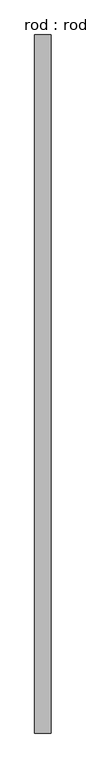
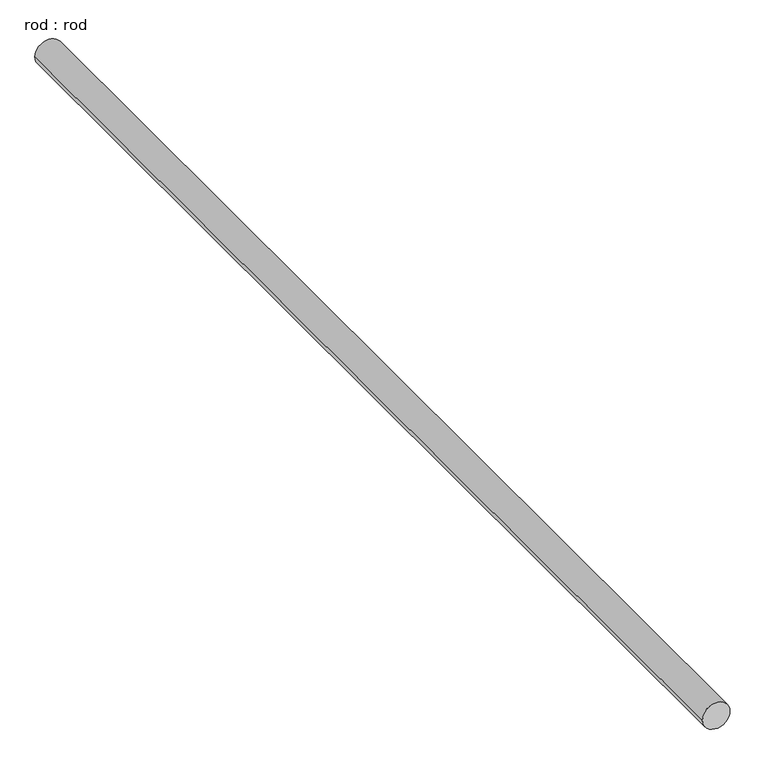
"""IFC4 building model written with IfcOpenShell, lengths in millimetres: proxy geometry, rod : rod."""

from ifc_helpers import new_model, si_unit, point, frame, frame_2d, origin, place, context, project, spatial, circle_curve, trimmed, segment, composite_curve, outline, extrude, source, transform, mapped, element, save


def rod_rod_caa43e47(model_context):
    return source(origin(), model_context, "Body", "SweptSolid", [
        extrude(outline(composite_curve([segment(trimmed(circle_curve(frame_2d((0.0108462, 0.0)), 200.0), [point((0.0108462, 200.0))], [point((0.0108462, -200.0))], False, "CARTESIAN"), True, "CONTINUOUS"), segment(trimmed(circle_curve(frame_2d((0.0108462, 0.0)), 200.0), [point((0.0108462, -200.0))], [point((0.0108462, 200.0))], False, "CARTESIAN"), True, "CONTINUOUS")], self_intersect=False)), frame((0.0, -4343.1908587, 0.0), z_axis=(0.0, 1.0, 0.0), x_axis=(0.0, 0.0, 1.0)), (0.0, 0.0, 1.0), 16871.8389481),
    ])


if __name__ == "__main__":
    model = new_model("IFC4")
    model_context = context("Model", 3, world=origin())
    ifc_project = project(units=[si_unit("LENGTHUNIT", "METRE", prefix="MILLI")], contexts=[model_context])
    site = spatial("IfcSite", under=ifc_project)
    building = spatial("IfcBuilding", under=site)
    placement = place(None, origin())
    rod_rod_shape = rod_rod_caa43e47(model_context)
    element("IfcBuildingElementProxy", 1, Name="rod : rod", ObjectType="rod : rod", at=placement, inside=building, context=model_context, shape_type="MappedRepresentation", body=[
        mapped(rod_rod_shape, transform((0.0, 0.0, 0.0), x_axis=(1.0, 0.0, 0.0), y_axis=(0.0, 1.0, 0.0), z_axis=(0.0, 0.0, 1.0))),
    ])
    save(model, "model.ifc")

# Revit data of these elements
# Type "rod : rod"
#   Default Elevation = 0
